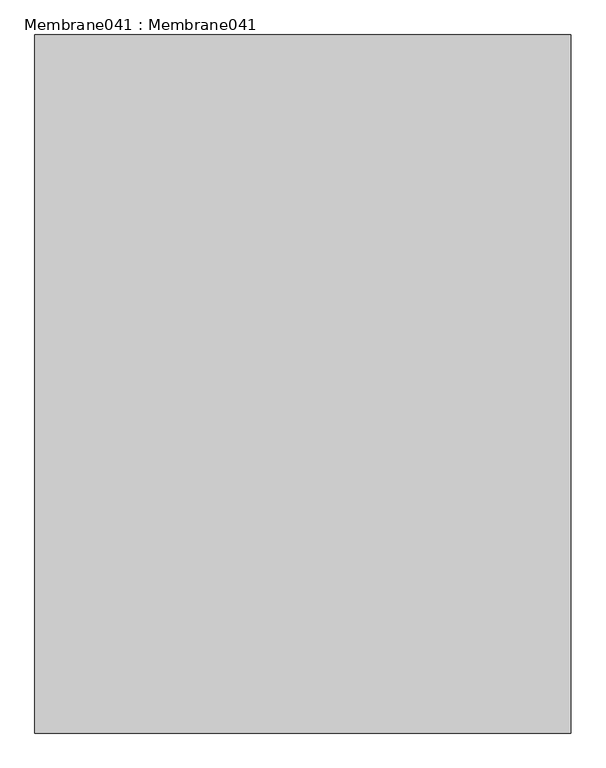
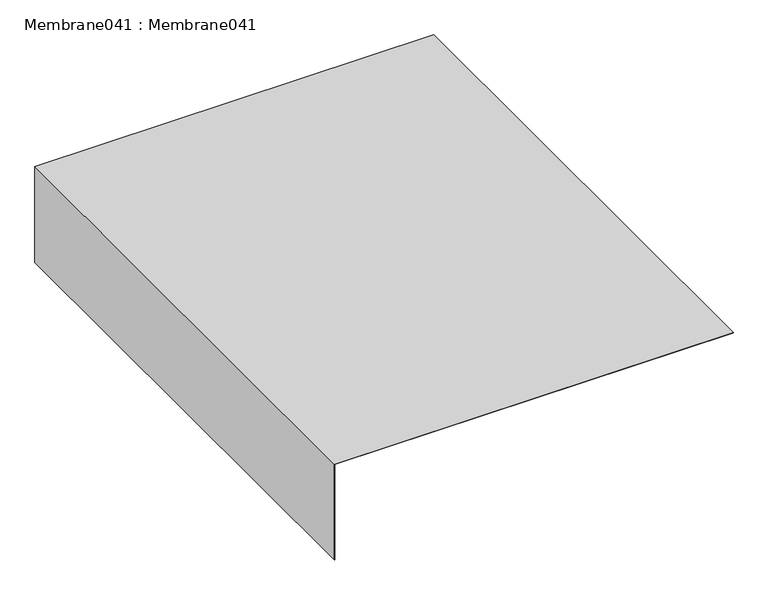
"""IFC4 building model written with IfcOpenShell, lengths in millimetres: proxy geometry, Membrane041 : Membrane041."""

from ifc_helpers import new_model, si_unit, frame, origin, place, context, project, spatial, polyline, outline, extrude, source, transform, mapped, element, save


def membrane041_membrane041_8a17b6ef(model_context):
    return source(origin(), model_context, "Body", "SweptSolid", [
        extrude(outline(polyline([(43443.8828125, -4953.168457), (43443.8828125, -6489.7270508), (43053.9921875, -6489.7270508), (43053.9921875, -6487.7270508), (43441.8828125, -6487.7270508), (43441.8828125, -4953.168457), (43443.8828125, -4953.168457)])), frame((0.0, 7982.1531721, 0.0), z_axis=(0.0, 1.0, 0.0), x_axis=(0.0, 0.0, 1.0)), (0.0, 0.0, 1.0), 2000.0),
    ])


if __name__ == "__main__":
    model = new_model("IFC4")
    model_context = context("Model", 3, world=origin())
    ifc_project = project(units=[si_unit("LENGTHUNIT", "METRE", prefix="MILLI")], contexts=[model_context])
    site = spatial("IfcSite", under=ifc_project)
    building = spatial("IfcBuilding", under=site)
    placement = place(None, origin())
    membrane041_membrane041_shape = membrane041_membrane041_8a17b6ef(model_context)
    element("IfcBuildingElementProxy", 1, Name="Membrane041 : Membrane041", ObjectType="Membrane041 : Membrane041", at=placement, inside=building, context=model_context, shape_type="MappedRepresentation", body=[
        mapped(membrane041_membrane041_shape, transform((0.0, 0.0, 0.0), x_axis=(1.0, 0.0, 0.0), y_axis=(0.0, 1.0, 0.0), z_axis=(0.0, 0.0, 1.0))),
    ])
    save(model, "model.ifc")

# Revit data of these elements
# Type "Membrane041 : Membrane041"
#   NameOverride = "Membrane041"
# Element 1 (IfcBuildingElementProxy, "Membrane041 : Membrane041")
#   Materials on its faces: "2 LAYERS NO. 30 ASTM D226 ASPHALT SATURATED ORGANIC FELT"
# Materials
#   "2 LAYERS NO. 30 ASTM D226 ASPHALT SATURATED ORGANIC FELT": class "Unassigned", colour RGB 46 171 0, transparency 0
